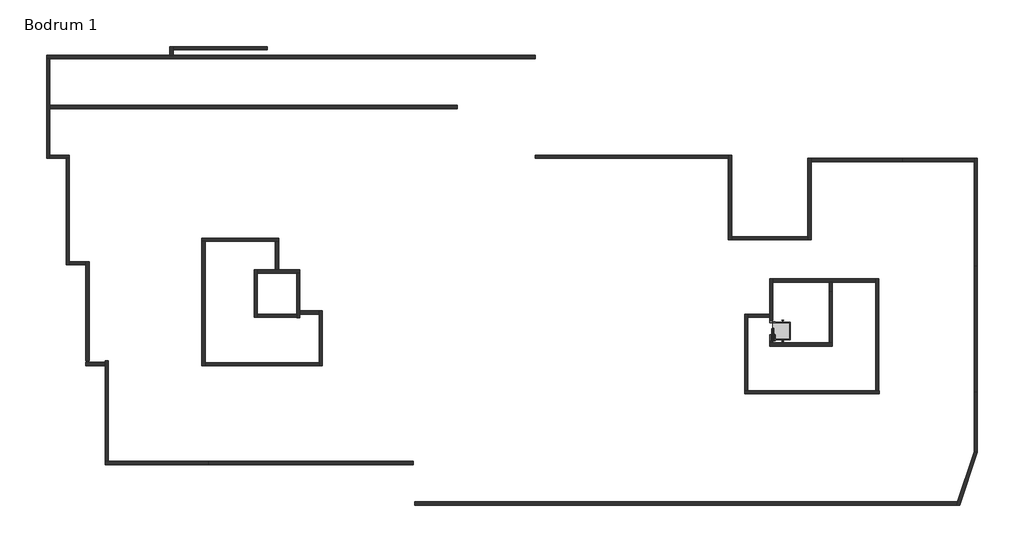
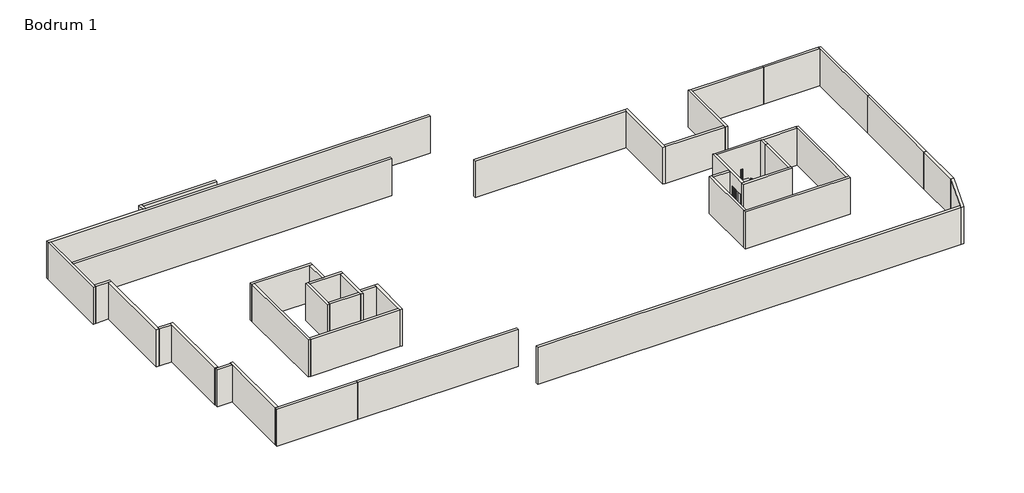
# One storey: 43 walls, 1 proxy.
"""IFC4 building model written with IfcOpenShell, lengths in millimetres."""

import ifcopenshell
import ifcopenshell.guid

model = None  # the IFC model being written
_history = None  # IfcOwnerHistory: only IFC2X3 demands one
_inside = {}  # id of a spatial element -> (the spatial element, [elements in it])
_under = {}  # id of a project, library or spatial element -> (it, [spatial elements below it])
_declared = {}  # id of a project -> (the project, [libraries it declares])
_typed = {}  # id of a type object -> (the type object, [elements of that type])
_made_of = {}  # id of a material, layer set ... -> (it, [elements and type objects made of it])


def new_model(schema):
    """Start an empty IFC model of exactly this schema.

    Asked for "IFC4X3", IfcOpenShell would pick the latest addendum, in which some entities
    have other attributes; the version numbers below select the first issue.
    IFC2X3 requires an IfcOwnerHistory on every rooted entity: one is made here for all.
    """
    global model, _history
    if schema == "IFC4X3":
        model = ifcopenshell.file(schema_version=(4, 3, 0, 0))
    else:
        model = ifcopenshell.file(schema=schema)
    _inside.clear()
    _under.clear()
    _declared.clear()
    _typed.clear()
    _made_of.clear()
    _history = None
    if model.schema == "IFC2X3":
        org = make("IfcOrganization", Name="unknown")
        user = make(
            "IfcPersonAndOrganization",
            ThePerson=make("IfcPerson", FamilyName="unknown"),
            TheOrganization=org,
        )
        app = make(
            "IfcApplication",
            ApplicationDeveloper=org,
            Version="unknown",
            ApplicationFullName="unknown",
            ApplicationIdentifier="unknown",
        )
        _history = make(
            "IfcOwnerHistory",
            OwningUser=user,
            OwningApplication=app,
            ChangeAction="ADDED",
            CreationDate=0,
        )
    return model


def make(cls, **values):
    """One entity of the class cls with the attributes given. An attribute that is None is left unset."""
    return model.create_entity(
        cls, **{name: value for name, value in values.items() if value is not None}
    )


def rooted(cls, **values):
    """An entity with a GlobalId (a new one), such as an element, a storey or a relation."""
    return make(cls, GlobalId=ifcopenshell.guid.new(), OwnerHistory=_history, **values)


def si_unit(unit_type, name, prefix=None):
    """IfcSIUnit, for example si_unit("LENGTHUNIT", "METRE", prefix="MILLI")."""
    return make("IfcSIUnit", UnitType=unit_type, Prefix=prefix, Name=name)


def assignment(units):
    """IfcUnitAssignment: the units of a project."""
    return None if units is None else make("IfcUnitAssignment", Units=units)


def point(xyz):
    """IfcCartesianPoint."""
    return None if xyz is None else make("IfcCartesianPoint", Coordinates=xyz)


def direction(xyz):
    """IfcDirection."""
    return None if xyz is None else make("IfcDirection", DirectionRatios=xyz)


def frame(location, z_axis=None, x_axis=None):
    """IfcAxis2Placement3D, a coordinate frame: its origin and axes. An axis left out is left unset."""
    return make(
        "IfcAxis2Placement3D",
        Location=point(location),
        Axis=direction(z_axis),
        RefDirection=direction(x_axis),
    )


def origin():
    """The frame at (0, 0, 0) with its axes left unset."""
    return frame((0.0, 0.0, 0.0))


def origin_with_axes():
    """The frame at (0, 0, 0) with the z axis (0, 0, 1) and the x axis (1, 0, 0) written out."""
    return frame((0.0, 0.0, 0.0), z_axis=(0.0, 0.0, 1.0), x_axis=(1.0, 0.0, 0.0))


def place(relative_to, where):
    """IfcLocalPlacement: puts the frame where relative to a parent placement (None: the world)."""
    return make(
        "IfcLocalPlacement", PlacementRelTo=relative_to, RelativePlacement=where
    )


def context(
    kind, dimensions, precision=None, world=None, true_north=None, identifier=None
):
    """IfcGeometricRepresentationContext, for example the 3D "Model" context."""
    return make(
        "IfcGeometricRepresentationContext",
        ContextIdentifier=identifier,
        ContextType=kind,
        CoordinateSpaceDimension=dimensions,
        Precision=precision,
        WorldCoordinateSystem=world,
        TrueNorth=true_north,
    )


def project(units=None, contexts=None):
    """IfcProject with its units and contexts."""
    return rooted(
        "IfcProject",
        Name="project",
        RepresentationContexts=contexts,
        UnitsInContext=assignment(units),
    )


def spatial(cls, under=None, at=None, **own):
    """A site, building, storey or space (cls), placed at a placement, below another one or the project."""
    s = rooted(cls, ObjectPlacement=at, **own)
    if under is not None:
        _under.setdefault(under.id(), (under, []))[1].append(s)
    return s


def polyline(points):
    """IfcPolyline through the points."""
    return make("IfcPolyline", Points=[point(p) for p in points])


def outline(outer, holes=None, kind="AREA"):
    """IfcArbitraryClosedProfileDef: a profile drawn as a closed curve; with holes, ...WithVoids."""
    if holes is None:
        return make("IfcArbitraryClosedProfileDef", ProfileType=kind, OuterCurve=outer)
    return make(
        "IfcArbitraryProfileDefWithVoids",
        ProfileType=kind,
        OuterCurve=outer,
        InnerCurves=holes,
    )


def extrude(swept, where, along, depth):
    """IfcExtrudedAreaSolid: the profile swept, set in the frame where, extruded along a direction by depth."""
    return make(
        "IfcExtrudedAreaSolid",
        SweptArea=swept,
        Position=where,
        ExtrudedDirection=direction(along),
        Depth=depth,
    )


def faces_of(points, faces, orient=None, outer=None):
    """IfcFace entities. A face is a list of loops; a loop is a list of indices into points, from 0.

    orient and outer hold one flag for each loop. By default every Orientation is true, the
    first loop of a face is its IfcFaceOuterBound and the others are IfcFaceBound.
    """
    made = []
    for i, loops in enumerate(faces):
        bounds = []
        for j, loop in enumerate(loops):
            is_outer = j == 0 if outer is None else outer[i][j]
            bounds.append(
                make(
                    "IfcFaceOuterBound" if is_outer else "IfcFaceBound",
                    Bound=make("IfcPolyLoop", Polygon=[points[k] for k in loop]),
                    Orientation=True if orient is None else orient[i][j],
                )
            )
        made.append(make("IfcFace", Bounds=bounds))
    return made


def faceted_brep(points, faces, orient=None, outer=None, voids=None):
    """IfcFacetedBrep: a solid bounded by flat faces; with voids (closed shells), ...WithVoids."""
    shared = [point(p) for p in points]
    hull = make("IfcClosedShell", CfsFaces=faces_of(shared, faces, orient, outer))
    if voids is None:
        return make("IfcFacetedBrep", Outer=hull)
    return make(
        "IfcFacetedBrepWithVoids",
        Outer=hull,
        Voids=[
            make(cls, CfsFaces=faces_of(shared, fs, o, b)) for cls, fs, o, b in voids
        ],
    )


def shape(context_of_items, identifier, shape_type, items):
    """IfcShapeRepresentation: the items that make up one representation, for example the "Body"."""
    return make(
        "IfcShapeRepresentation",
        ContextOfItems=context_of_items,
        RepresentationIdentifier=identifier,
        RepresentationType=shape_type,
        Items=items,
    )


def source(mapping_origin, context_of_items, identifier, shape_type, items):
    """IfcRepresentationMap: a shape defined once, which mapped items show again and again."""
    return make(
        "IfcRepresentationMap",
        MappingOrigin=mapping_origin,
        MappedRepresentation=shape(context_of_items, identifier, shape_type, items),
    )


def transform(
    local_origin,
    x_axis=None,
    y_axis=None,
    z_axis=None,
    scale=None,
    scale2=None,
    scale3=None,
    uniform=True,
):
    """IfcCartesianTransformationOperator3D, or its non-uniform kind. x_axis, y_axis, z_axis: its Axis1, 2, 3."""
    if uniform:
        return make(
            "IfcCartesianTransformationOperator3D",
            Axis1=direction(x_axis),
            Axis2=direction(y_axis),
            LocalOrigin=point(local_origin),
            Scale=scale,
            Axis3=direction(z_axis),
        )
    return make(
        "IfcCartesianTransformationOperator3DnonUniform",
        Axis1=direction(x_axis),
        Axis2=direction(y_axis),
        LocalOrigin=point(local_origin),
        Scale=scale,
        Axis3=direction(z_axis),
        Scale2=scale2,
        Scale3=scale3,
    )


def mapped(mapping_source, mapping_target):
    """IfcMappedItem: shows the shape of a source again, moved by a transform."""
    return make(
        "IfcMappedItem", MappingSource=mapping_source, MappingTarget=mapping_target
    )


def made_of(thing, what):
    """Note that an element or type object is made of a material, layer set ...; save() writes the relation."""
    if what is not None:
        _made_of.setdefault(what.id(), (what, []))[1].append(thing)
    return thing


def element(
    cls,
    number,
    at=None,
    inside=None,
    cuts=None,
    type_object=None,
    material=None,
    context=None,
    identifier="Body",
    shape_type=None,
    held_by="IfcProductDefinitionShape",
    body=None,
    shapes=None,
    **own,
):
    """One element of the class cls, such as IfcWall. Its Tag is "e" and its number.

    at: its placement. inside: the storey or other place that contains it. cuts: it is an
    opening in that element (IfcRelVoidsElement). A single representation is given by context,
    identifier, shape_type and body (its items); several are given by shapes. held_by: the class
    of the entity that holds the representations. save() writes the other relations.
    """
    e = rooted(cls, Tag="e%d" % number, ObjectPlacement=at, **own)
    if body is not None:
        shapes = [shape(context, identifier, shape_type, body)]
    if shapes is not None:
        e.Representation = make(held_by, Representations=shapes)
    if inside is not None:
        _inside.setdefault(inside.id(), (inside, []))[1].append(e)
    if cuts is not None:
        rooted(
            "IfcRelVoidsElement", RelatingBuildingElement=cuts, RelatedOpeningElement=e
        )
    if type_object is not None:
        _typed.setdefault(type_object.id(), (type_object, []))[1].append(e)
    return made_of(e, material)


def aggregate(whole, parts):
    """IfcRelAggregates: a whole, such as a stair, and the parts it consists of."""
    return rooted("IfcRelAggregates", RelatingObject=whole, RelatedObjects=parts)


def save(model, path):
    """Write the relations noted so far, then the file.

    IfcRelAggregates (storeys below a building ...), IfcRelContainedInSpatialStructure (elements
    in a storey), IfcRelDefinesByType, IfcRelAssociatesMaterial and IfcRelDeclares: one each for
    every whole, place, type object, material and project.
    """
    for whole, parts in _under.values():
        aggregate(whole, parts)
    for where, things in _inside.values():
        rooted(
            "IfcRelContainedInSpatialStructure",
            RelatedElements=things,
            RelatingStructure=where,
        )
    for kind, things in _typed.values():
        rooted("IfcRelDefinesByType", RelatedObjects=things, RelatingType=kind)
    for what, things in _made_of.values():
        rooted("IfcRelAssociatesMaterial", RelatedObjects=things, RelatingMaterial=what)
    for by, libraries in _declared.values():
        rooted("IfcRelDeclares", RelatingContext=by, RelatedDefinitions=libraries)
    model.write(path)


def m_electric_lift_4_person_wall_based_type_1_25105fba(model_context):
    return source(origin(), model_context, "Body", "SolidModel", [
        extrude(outline(polyline([(-400.0, -1140.0000001), (-400.0, -235.0), (-486.5, -235.0), (-486.5, -105.0), (681.0, -105.0), (681.0, -235.0), (650.0, -235.0), (650.0, -1140.0000001), (-400.0, -1140.0000001)])), frame((0.0, 0.0, 2200.0), z_axis=(0.0, 0.0, 1.0), x_axis=(1.0, 0.0, 0.0)), (0.0, 0.0, 1.0), 22.0),
        extrude(outline(polyline([(-448.6220553, -190.9893804), (-448.6220553, -149.3893804), (-62.6220553, -149.3893804), (-62.6220553, -190.9893804), (-448.6220553, -190.9893804)])), origin_with_axes(), (0.0, 0.0, 1.0), 2000.0),
        extrude(outline(polyline([(-114.8301, -144.0), (-114.8301, -108.9587126), (271.1699, -108.9587126), (271.1699, -144.0), (-114.8301, -144.0)])), origin_with_axes(), (0.0, 0.0, 1.0), 2000.0),
        extrude(outline(polyline([(-488.6220553, 8.3893803), (-102.6220553, 8.3893803), (-102.6220553, -30.6106197), (-488.6220553, -30.6106197), (-488.6220553, 8.3893803)])), origin_with_axes(), (0.0, 0.0, 1.0), 2000.0),
        extrude(outline(polyline([(-124.8301, -75.0), (-124.8301, -36.0), (261.1699, -36.0), (261.1699, -75.0), (-124.8301, -75.0)])), origin_with_axes(), (0.0, 0.0, 1.0), 2000.0),
        extrude(outline(polyline([(-400.0, -1140.0000001), (-400.0, -235.0), (-486.5, -235.0), (-486.5, -105.0), (681.0, -105.0), (681.0, -235.0), (650.0, -235.0), (650.0, -1140.0000001), (-400.0, -1140.0000001)])), frame((0.0, 0.0, -90.0), z_axis=(0.0, 0.0, 1.0), x_axis=(1.0, 0.0, 0.0)), (0.0, 0.0, 1.0), 90.0),
        faceted_brep([(-400.0, -1140.0000001, 2200.0), (650.0, -1140.0000001, 2200.0), (650.0, -235.0, 2200.0), (681.0, -235.0, 2200.0), (681.0, -105.0, 2200.0), (-486.5, -105.0, 2200.0), (-486.5, -235.0, 2200.0), (-400.0, -235.0, 2200.0), (-375.0, -1115.0000001, 2200.0), (-375.0, -235.0, 2200.0), (-110.3, -235.0, 2200.0), (-110.3, -197.0, 2200.0), (-458.1228936, -197.0, 2200.0), (-458.1228936, -108.9587126, 2200.0), (621.1699, -108.9587126, 2200.0), (621.1699, -192.6835257, 2200.0), (600.0, -192.6835257, 2200.0), (600.0, -235.0, 2200.0), (625.0, -235.0, 2200.0), (625.0, -572.5016433, 2200.0), (610.2454439, -572.5016433, 2200.0), (610.2454439, -802.5016433, 2200.0), (625.0, -802.5016433, 2200.0), (625.0, -1115.0000001, 2200.0), (-400.0, -1140.0000001, 0.0), (-400.0, -235.0, 0.0), (-486.5, -235.0, 0.0), (-486.5, -105.0, 0.0), (-173.4437103, -105.0, 0.0), (-173.4437103, -108.9587126, 0.0), (-458.1228936, -108.9587126, 0.0), (-458.1228936, -197.0, 0.0), (-110.3, -197.0, 0.0), (-110.3, -235.0, 0.0), (-375.0, -235.0, 0.0), (-375.0, -1115.0000001, 0.0), (625.0, -1115.0000001, 0.0), (625.0, -802.5016433, 0.0), (610.2454439, -802.5016433, 0.0), (610.2454439, -572.5016433, 0.0), (625.0, -572.5016433, 0.0), (625.0, -235.0, 0.0), (600.0, -235.0, 0.0), (600.0, -192.6835257, 0.0), (621.1699, -192.6835257, 0.0), (621.1699, -105.0, 0.0), (681.0, -105.0, 0.0), (681.0, -235.0, 0.0), (650.0, -235.0, 0.0), (650.0, -1140.0000001, 0.0), (621.1699, -105.0, 2000.0), (-173.4437103, -105.0, 2000.0), (-173.4437103, -108.9587126, 2000.0), (621.1699, -108.9587126, 2000.0), (600.0, -192.6835257, 2000.0)], [[[0, 1, 2, 3, 4, 5, 6, 7], [8, 9, 10, 11, 12, 13, 14, 15, 16, 17, 18, 19, 20, 21, 22, 23]], [[24, 25, 26, 27, 28, 29, 30, 31, 32, 33, 34, 35, 36, 37, 38, 39, 40, 41, 42, 43, 44, 45, 46, 47, 48, 49]], [[1, 0, 24, 49]], [[2, 1, 49, 48]], [[3, 2, 48, 47]], [[4, 3, 47, 46]], [[5, 4, 46, 45, 50, 51, 28, 27]], [[6, 5, 27, 26]], [[7, 6, 26, 25]], [[0, 7, 25, 24]], [[9, 8, 35, 34]], [[10, 9, 34, 33]], [[11, 10, 33, 32]], [[12, 11, 32, 31]], [[13, 12, 31, 30]], [[14, 13, 30, 29, 52, 53]], [[15, 14, 53, 50, 45, 44]], [[16, 15, 44, 43, 54]], [[17, 16, 54, 43, 42]], [[18, 17, 42, 41]], [[19, 18, 41, 40]], [[20, 19, 40, 39]], [[21, 20, 39, 38]], [[22, 21, 38, 37]], [[23, 22, 37, 36]], [[8, 23, 36, 35]], [[50, 53, 52, 51]], [[51, 52, 29, 28]]]),
        extrude(outline(polyline([(750.026988, -751.0012199), (747.026988, -693.80122), (682.0269884, -693.80122), (682.0269884, -681.3056039), (747.1132057, -681.3056039), (750.026988, -624.0012199), (763.026988, -624.0012199), (763.026988, -751.0012199), (750.026988, -751.0012199)])), origin_with_axes(), (0.0, 0.0, 1.0), 3000.0),
        extrude(outline(polyline([(-497.026988, -693.80122), (-500.026988, -751.0012199), (-513.026988, -751.0012199), (-513.026988, -624.0012199), (-500.026988, -624.0012199), (-497.1132057, -681.3056039), (-432.0269884, -681.3056039), (-432.0269884, -693.80122), (-497.026988, -693.80122)])), origin_with_axes(), (0.0, 0.0, 1.0), 3000.0),
        extrude(outline(polyline([(-114.9791786, 100.0), (-114.9791786, 14.4785696), (-505.0067971, 14.4785696), (-505.0067971, 100.0), (-114.9791786, 100.0)])), origin_with_axes(), (0.0, 0.0, 1.0), 2000.0),
        extrude(outline(polyline([(600.0, 5.0), (600.0, 100.0), (750.0, 100.0), (750.0, -75.0), (621.1699, -75.0), (621.1699, 5.0), (600.0, 5.0)])), origin_with_axes(), (0.0, 0.0, 1.0), 2000.0),
    ])


model = new_model("IFC4")

# Units and contexts
model_context = context("Model", 3, world=origin())
ifc_project = project(units=[si_unit("LENGTHUNIT", "METRE", prefix="MILLI")], contexts=[model_context])

# Site, building, storey
site = spatial("IfcSite", under=ifc_project)
building = spatial("IfcBuilding", under=site)
storey = spatial("IfcBuildingStorey", under=building, Name="Bodrum 1", Elevation=-3000.0)

# Proxy
placement = place(None, origin())
m_electric_lift_4_person_wall_based_type_1_shape = m_electric_lift_4_person_wall_based_type_1_25105fba(model_context)
element("IfcBuildingElementProxy", 1, Name="M_Electric Lift-4 person wall based : Type 1", ObjectType="M_Electric Lift-4 person wall based : Type 1", at=placement, inside=storey, context=model_context, shape_type="MappedRepresentation", body=[
    mapped(m_electric_lift_4_person_wall_based_type_1_shape, transform((17860.0831827, -2691.3136213, -3000.0), x_axis=(0.0, 1.0, 0.0), y_axis=(-1.0, 0.0, 0.0), z_axis=(0.0, 0.0, 1.0))),
])

# Walls
element("IfcWall", 2, ObjectType="Generic - 200mm", at=placement, inside=storey, context=model_context, shape_type="SweptSolid", body=[
    extrude(outline(polyline([(30057.8216012, 7604.4428324), (25739.3154183, 7604.4428324), (25739.3154183, 7804.4428324), (30057.8216012, 7804.4428324), (30057.8216012, 7604.4428324)])), frame((0.0, 0.0, -3000.0), z_axis=(0.0, 0.0, 1.0), x_axis=(1.0, 0.0, 0.0)), (0.0, 0.0, 1.0), 3000.0),
])
element("IfcWall", 3, ObjectType="Generic - 200mm", at=placement, inside=storey, context=model_context, shape_type="Brep", body=[
    faceted_brep([(30057.8216012, 7804.4428324, -3000.0), (30057.8216012, 7604.4428324, -3000.0), (30057.8216012, 1304.4428324, -3000.0), (30057.8216012, 1304.4428324, 0.0), (30057.8216012, 7604.4428324, 0.0), (30057.8216012, 7804.4428324, 0.0), (30257.8216012, 7804.4428324, -3000.0), (30257.8216012, 7804.4428324, 0.0), (30257.8216012, 1304.4428324, 0.0), (30257.8216012, 1304.4428324, -3000.0), (30058.3403162, 1304.4428324, -3000.0), (30058.3403162, 1304.4428324, 0.0)], [[[0, 1, 2, 3, 4, 5]], [[6, 7, 8, 9]], [[2, 1, 0, 6, 9, 10]], [[3, 2, 10, 9, 8, 11]], [[5, 4, 3, 11, 8, 7]], [[0, 5, 7, 6]]]),
])
element("IfcWall", 4, ObjectType="Generic - 200mm", at=placement, inside=storey, context=model_context, shape_type="Brep", body=[
    faceted_brep([(30058.3403162, 1304.4428324, -3000.0), (30058.3403162, -6255.0426075, -3000.0), (30058.3403162, -6255.0426075, 0.0), (30058.3403162, 1304.4428324, 0.0), (30258.3403162, 1304.4428324, -3000.0), (30258.3403162, 1304.4428324, 0.0), (30258.3403162, -6255.0426075, 0.0), (30258.3403162, -6255.0426075, -3000.0), (30257.8216012, 1304.4428324, -3000.0), (30058.8590312, -6255.0426075, -3000.0), (30058.8590312, -6255.0426075, 0.0), (30257.8216012, 1304.4428324, 0.0)], [[[0, 1, 2, 3]], [[4, 5, 6, 7]], [[1, 0, 8, 4, 7, 9]], [[2, 1, 9, 7, 6, 10]], [[3, 2, 10, 6, 5, 11]], [[0, 3, 11, 5, 4, 8]]]),
])
element("IfcWall", 5, ObjectType="Generic - 200mm", at=placement, inside=storey, context=model_context, shape_type="Brep", body=[
    faceted_brep([(30058.8590312, -6255.0426075, -3000.0), (30058.8590312, -9846.9059148, -3000.0), (30058.8590312, -9846.9059148, 0.0), (30058.8590312, -6255.0426075, 0.0), (30258.8590312, -6255.0426075, -3000.0), (30258.8590312, -6255.0426075, 0.0), (30258.8590312, -9879.7441648, 0.0), (30258.8590312, -9879.7441648, -3000.0), (30258.3403162, -6255.0426075, -3000.0), (30258.3403162, -6255.0426075, 0.0)], [[[0, 1, 2, 3]], [[4, 5, 6, 7]], [[1, 0, 8, 4, 7]], [[3, 2, 6, 5, 9]], [[0, 3, 9, 5, 4, 8]], [[2, 1, 7, 6]]]),
])
element("IfcWall", 6, ObjectType="Generic - 200mm", at=placement, inside=storey, context=model_context, shape_type="Brep", body=[
    faceted_brep([(21539.3154183, -3291.3136212, -3000.0), (21339.3154183, -3291.3136212, -3000.0), (17960.0831827, -3291.3136212, -3000.0), (17760.0831827, -3291.3136212, -3000.0), (17760.0831827, -3291.3136212, 0.0), (17960.0831827, -3291.3136212, 0.0), (21339.3154183, -3291.3136212, 0.0), (21539.3154183, -3291.3136212, 0.0), (21539.3154183, -3491.3136212, -3000.0), (21539.3154183, -3491.3136212, 0.0), (17760.0831827, -3491.3136212, 0.0), (17760.0831827, -3491.3136212, -3000.0)], [[[0, 1, 2, 3, 4, 5, 6, 7]], [[8, 9, 10, 11]], [[3, 2, 1, 0, 8, 11]], [[7, 6, 5, 4, 10, 9]], [[0, 7, 9, 8]], [[4, 3, 11, 10]]]),
])
element("IfcWall", 7, ObjectType="Generic - 200mm", at=placement, inside=storey, context=model_context, shape_type="SweptSolid", body=[
    extrude(outline(polyline([(-3560.351342, -12851.723579), (29044.7914835, -12851.723579), (28977.2953715, -13051.723579), (-3560.351342, -13051.723579), (-3560.351342, -12851.723579)])), frame((0.0, 0.0, -3000.0), z_axis=(0.0, 0.0, 1.0), x_axis=(1.0, 0.0, 0.0)), (0.0, 0.0, 1.0), 3000.0),
])
element("IfcWall", 8, ObjectType="Generic - 200mm", at=placement, inside=storey, context=model_context, shape_type="Brep", body=[
    faceted_brep([(30058.8590312, -9846.9059148, -3000.0), (29044.7914835, -12851.723579, -3000.0), (28977.2953715, -13051.723579, -3000.0), (28977.2953715, -13051.723579, 0.0), (29044.7914835, -12851.723579, 0.0), (30058.8590312, -9846.9059148, 0.0), (30258.8590312, -9879.7441648, -3000.0), (30258.8590312, -9879.7441648, 0.0), (29188.3776425, -13051.723579, 0.0), (29188.3776425, -13051.723579, -3000.0)], [[[0, 1, 2, 3, 4, 5]], [[6, 7, 8, 9]], [[2, 1, 0, 6, 9]], [[5, 4, 3, 8, 7]], [[0, 5, 7, 6]], [[3, 2, 9, 8]]]),
])
element("IfcWall", 9, ObjectType="Generic - 200mm", at=placement, inside=storey, context=model_context, shape_type="Brep", body=[
    faceted_brep([(24352.8789167, -6155.0426075, -3000.0), (24338.3403162, -6155.0426075, -3000.0), (24138.3403162, -6155.0426075, -3000.0), (16460.0831827, -6155.0426075, -3000.0), (16260.0831827, -6155.0426075, -3000.0), (16260.0831827, -6155.0426075, 0.0), (16460.0831827, -6155.0426075, 0.0), (24138.3403162, -6155.0426075, 0.0), (24338.3403162, -6155.0426075, 0.0), (24352.8789167, -6155.0426075, 0.0), (24352.8789167, -6355.0426075, -3000.0), (24352.8789167, -6355.0426075, 0.0), (16260.0831827, -6355.0426075, 0.0), (16260.0831827, -6355.0426075, -3000.0)], [[[0, 1, 2, 3, 4, 5, 6, 7, 8, 9]], [[10, 11, 12, 13]], [[4, 3, 2, 1, 0, 10, 13]], [[9, 8, 7, 6, 5, 12, 11]], [[0, 9, 11, 10]], [[5, 4, 13, 12]]]),
])
element("IfcWall", 10, ObjectType="Generic - 200mm", at=placement, inside=storey, context=model_context, shape_type="Brep", body=[
    faceted_brep([(24338.3403162, -6155.0426075, -3000.0), (24338.3403162, 564.4428324, -3000.0), (24338.3403162, 564.4428324, 0.0), (24338.3403162, -6155.0426075, 0.0), (24138.3403162, -6155.0426075, -3000.0), (24138.3403162, -6155.0426075, 0.0), (24138.3403162, 364.4428324, 0.0), (24138.3403162, 564.4428324, 0.0), (24138.3403162, 564.4428324, -3000.0), (24138.3403162, 364.4428324, -3000.0)], [[[0, 1, 2, 3]], [[4, 5, 6, 7, 8, 9]], [[1, 0, 4, 9, 8]], [[3, 2, 7, 6, 5]], [[0, 3, 5, 4]], [[2, 1, 8, 7]]]),
])
element("IfcWall", 11, ObjectType="Generic - 200mm", at=placement, inside=storey, context=model_context, shape_type="SweptSolid", body=[
    extrude(outline(polyline([(21339.3154183, -3291.3136212), (21339.3154183, -215.5571676), (21539.3154183, -215.5571676), (21539.3154183, -3291.3136212), (21339.3154183, -3291.3136212)])), frame((0.0, 0.0, -3000.0), z_axis=(0.0, 0.0, 1.0), x_axis=(1.0, 0.0, 0.0)), (0.0, 0.0, 1.0), 3000.0),
])
element("IfcWall", 12, ObjectType="Generic - 200mm", at=placement, inside=storey, context=model_context, shape_type="Brep", body=[
    faceted_brep([(17760.0831827, -3291.3136212, 0.0), (17760.0831827, -1755.0426075, 0.0), (17760.0831827, -1555.0426075, 0.0), (17760.0831827, 564.4428324, 0.0), (17760.0831827, 564.4428324, -3000.0), (17760.0831827, -1555.0426075, -3000.0), (17760.0831827, -1755.0426075, -3000.0), (17760.0831827, -1941.3136213, -3000.0), (17760.0831827, -1941.3136213, -1000.0), (17760.0831827, -3196.3204184, -1000.0), (17760.0831827, -3196.3204184, -3000.0), (17760.0831827, -3291.3136212, -3000.0), (17960.0831827, 564.4428324, 0.0), (17960.0831827, 364.4428324, 0.0), (17960.0831827, -3291.3136212, 0.0), (17960.0831827, -3291.3136212, -3000.0), (17960.0831827, -3196.3204184, -3000.0), (17960.0831827, -3196.3204184, -1000.0), (17960.0831827, -1941.3136213, -1000.0), (17960.0831827, -1941.3136213, -3000.0), (17960.0831827, 364.4428324, -3000.0), (17960.0831827, 564.4428324, -3000.0)], [[[0, 1, 2, 3, 4, 5, 6, 7, 8, 9, 10, 11]], [[12, 13, 14, 15, 16, 17, 18, 19, 20, 21]], [[15, 11, 10, 16]], [[4, 21, 20, 19, 7, 6, 5]], [[3, 2, 1, 0, 14, 13, 12]], [[0, 11, 15, 14]], [[9, 17, 16, 10]], [[18, 8, 7, 19]], [[8, 18, 17, 9]], [[21, 4, 3, 12]]]),
])
element("IfcWall", 13, ObjectType="Generic - 200mm", at=placement, inside=storey, context=model_context, shape_type="SweptSolid", body=[
    extrude(outline(polyline([(21539.3154183, 364.4428324), (21539.3154183, -215.5571676), (21339.3154183, -215.5571676), (21339.3154183, 364.4428324), (21539.3154183, 364.4428324)])), frame((0.0, 0.0, -3000.0), z_axis=(0.0, 0.0, 1.0), x_axis=(1.0, 0.0, 0.0)), (0.0, 0.0, 1.0), 3000.0),
])
element("IfcWall", 14, ObjectType="Generic - 200mm", at=placement, inside=storey, context=model_context, shape_type="SweptSolid", body=[
    extrude(outline(polyline([(25739.3154183, 7604.4428324), (20258.3403162, 7604.4428324), (20258.3403162, 7804.4428324), (25739.3154183, 7804.4428324), (25739.3154183, 7604.4428324)])), frame((0.0, 0.0, -3000.0), z_axis=(0.0, 0.0, 1.0), x_axis=(1.0, 0.0, 0.0)), (0.0, 0.0, 1.0), 3000.0),
])
element("IfcWall", 15, ObjectType="Generic - 200mm", at=placement, inside=storey, context=model_context, shape_type="Brep", body=[
    faceted_brep([(16460.0831827, -6155.0426075, -3000.0), (16460.0831827, -1755.0426075, -3000.0), (16460.0831827, -1555.0426075, -3000.0), (16460.0831827, -1555.0426075, 0.0), (16460.0831827, -1755.0426075, 0.0), (16460.0831827, -6155.0426075, 0.0), (16260.0831827, -6155.0426075, -3000.0), (16260.0831827, -6155.0426075, 0.0), (16260.0831827, -1555.0426075, 0.0), (16260.0831827, -1555.0426075, -3000.0)], [[[0, 1, 2, 3, 4, 5]], [[6, 7, 8, 9]], [[2, 1, 0, 6, 9]], [[5, 4, 3, 8, 7]], [[3, 2, 9, 8]], [[0, 5, 7, 6]]]),
])
element("IfcWall", 16, ObjectType="Generic - 200mm", at=placement, inside=storey, context=model_context, shape_type="Brep", body=[
    faceted_brep([(20058.3403162, 7804.4428324, -3000.0), (20058.3403162, 3104.4428324, -3000.0), (20058.3403162, 2904.4428324, -3000.0), (20058.3403162, 2904.4428324, 0.0), (20058.3403162, 3104.4428324, 0.0), (20058.3403162, 7804.4428324, 0.0), (20258.3403162, 7804.4428324, -3000.0), (20258.3403162, 7804.4428324, 0.0), (20258.3403162, 7604.4428324, 0.0), (20258.3403162, 2904.4428324, 0.0), (20258.3403162, 2904.4428324, -3000.0), (20258.3403162, 7604.4428324, -3000.0)], [[[0, 1, 2, 3, 4, 5]], [[6, 7, 8, 9, 10, 11]], [[2, 1, 0, 6, 11, 10]], [[5, 4, 3, 9, 8, 7]], [[0, 5, 7, 6]], [[3, 2, 10, 9]]]),
])
element("IfcWall", 17, ObjectType="Generic - 200mm", at=placement, inside=storey, context=model_context, shape_type="Brep", body=[
    faceted_brep([(24138.3403162, 564.4428324, -3000.0), (17960.0831827, 564.4428324, -3000.0), (17960.0831827, 564.4428324, 0.0), (24138.3403162, 564.4428324, 0.0), (24138.3403162, 364.4428324, -3000.0), (24138.3403162, 364.4428324, 0.0), (21539.3154183, 364.4428324, 0.0), (21339.3154183, 364.4428324, 0.0), (17960.0831827, 364.4428324, 0.0), (17960.0831827, 364.4428324, -3000.0), (21339.3154183, 364.4428324, -3000.0), (21539.3154183, 364.4428324, -3000.0)], [[[0, 1, 2, 3]], [[4, 5, 6, 7, 8, 9, 10, 11]], [[1, 0, 4, 11, 10, 9]], [[3, 2, 8, 7, 6, 5]], [[2, 1, 9, 8]], [[0, 3, 5, 4]]]),
])
element("IfcWall", 18, ObjectType="Generic - 200mm", at=placement, inside=storey, context=model_context, shape_type="Brep", body=[
    faceted_brep([(-3649.8304233, -10404.1955085, -3000.0), (-15985.351342, -10404.1955085, -3000.0), (-15985.351342, -10404.1955085, 0.0), (-3649.8304233, -10404.1955085, 0.0), (-3649.8304233, -10604.1955085, -3000.0), (-3649.8304233, -10604.1955085, 0.0), (-15985.351342, -10604.1955085, 0.0), (-15985.351342, -10604.1955085, -3000.0), (-15985.351342, -10404.7142235, -3000.0), (-15985.351342, -10404.7142235, 0.0)], [[[0, 1, 2, 3]], [[4, 5, 6, 7]], [[1, 0, 4, 7, 8]], [[2, 1, 8, 7, 6, 9]], [[3, 2, 9, 6, 5]], [[0, 3, 5, 4]]]),
])
element("IfcWall", 19, ObjectType="Generic - 200mm", at=placement, inside=storey, context=model_context, shape_type="Brep", body=[
    faceted_brep([(-15985.351342, -10404.7142235, -3000.0), (-21996.1656446, -10404.7142235, -3000.0), (-22196.1656446, -10404.7142235, -3000.0), (-22196.1656446, -10404.7142235, 0.0), (-21996.1656446, -10404.7142235, 0.0), (-15985.351342, -10404.7142235, 0.0), (-15985.351342, -10604.7142235, -3000.0), (-15985.351342, -10604.7142235, 0.0), (-22196.1656446, -10604.7142235, 0.0), (-22196.1656446, -10604.7142235, -3000.0), (-15985.351342, -10604.1955085, -3000.0), (-15985.351342, -10604.1955085, 0.0)], [[[0, 1, 2, 3, 4, 5]], [[6, 7, 8, 9]], [[2, 1, 0, 10, 6, 9]], [[5, 4, 3, 8, 7, 11]], [[0, 5, 11, 7, 6, 10]], [[3, 2, 9, 8]]]),
])
element("IfcWall", 20, ObjectType="Generic - 200mm", at=placement, inside=storey, context=model_context, shape_type="Brep", body=[
    faceted_brep([(-13036.6223557, -1755.1706106, -3000.0), (-13036.6223557, -1555.1706106, -3000.0), (-13036.6223557, 905.8044915, -3000.0), (-13036.6223557, 1105.8044915, -3000.0), (-13036.6223557, 1105.8044915, 0.0), (-13036.6223557, 905.8044915, 0.0), (-13036.6223557, -1555.1706106, 0.0), (-13036.6223557, -1755.1706106, 0.0), (-13236.6223557, -1755.1706106, -3000.0), (-13236.6223557, -1755.1706106, 0.0), (-13236.6223557, 1105.8044915, 0.0), (-13236.6223557, 1105.8044915, -3000.0)], [[[0, 1, 2, 3, 4, 5, 6, 7]], [[8, 9, 10, 11]], [[3, 2, 1, 0, 8, 11]], [[7, 6, 5, 4, 10, 9]], [[0, 7, 9, 8]], [[4, 3, 11, 10]]]),
])
element("IfcWall", 21, ObjectType="Generic - 200mm", at=placement, inside=storey, context=model_context, shape_type="Brep", body=[
    faceted_brep([(-23157.0323135, -4360.3976601, -3000.0), (-23157.0323135, 1599.6023399, -3000.0), (-23157.0323135, 1599.6023399, 0.0), (-23157.0323135, -4360.3976601, 0.0), (-23357.0323135, -4360.3976601, -3000.0), (-23357.0323135, -4360.3976601, 0.0), (-23357.0323135, 1399.6023399, 0.0), (-23357.0323135, 1599.6023399, 0.0), (-23357.0323135, 1599.6023399, -3000.0), (-23357.0323135, 1399.6023399, -3000.0)], [[[0, 1, 2, 3]], [[4, 5, 6, 7, 8, 9]], [[1, 0, 4, 9, 8]], [[3, 2, 7, 6, 5]], [[0, 3, 5, 4]], [[2, 1, 8, 7]]]),
])
element("IfcWall", 22, ObjectType="Generic - 200mm", at=placement, inside=storey, context=model_context, shape_type="Brep", body=[
    faceted_brep([(-16184.4950909, -4674.1955085, -3000.0), (-16184.4950909, -4474.1955085, -3000.0), (-16184.4950909, 2805.8044915, -3000.0), (-16184.4950909, 2805.8044915, 0.0), (-16184.4950909, -4474.1955085, 0.0), (-16184.4950909, -4674.1955085, 0.0), (-16384.4950909, -4674.1955085, -3000.0), (-16384.4950909, -4674.1955085, 0.0), (-16384.4950909, 2805.8044915, 0.0), (-16384.4950909, 2805.8044915, -3000.0)], [[[0, 1, 2, 3, 4, 5]], [[6, 7, 8, 9]], [[2, 1, 0, 6, 9]], [[5, 4, 3, 8, 7]], [[3, 2, 9, 8]], [[0, 5, 7, 6]]]),
])
element("IfcWall", 23, ObjectType="Generic - 200mm", at=placement, inside=storey, context=model_context, shape_type="SweptSolid", body=[
    extrude(outline(polyline([(-9320.909351, -4674.1955085), (-16184.4950909, -4674.1955085), (-16184.4950909, -4474.1955085), (-9320.909351, -4474.1955085), (-9320.909351, -4674.1955085)])), frame((0.0, 0.0, -3000.0), z_axis=(0.0, 0.0, 1.0), x_axis=(1.0, 0.0, 0.0)), (0.0, 0.0, 1.0), 3000.0),
])
element("IfcWall", 24, ObjectType="Generic - 200mm", at=placement, inside=storey, context=model_context, shape_type="SweptSolid", body=[
    extrude(outline(polyline([(-13036.6223557, -1555.1706106), (-10680.351342, -1555.1706106), (-10680.351342, -1755.1706106), (-13036.6223557, -1755.1706106), (-13036.6223557, -1555.1706106)])), frame((0.0, 0.0, -3000.0), z_axis=(0.0, 0.0, 1.0), x_axis=(1.0, 0.0, 0.0)), (0.0, 0.0, 1.0), 3000.0),
])
element("IfcWall", 25, ObjectType="Generic - 200mm", at=placement, inside=storey, context=model_context, shape_type="Brep", body=[
    faceted_brep([(-10480.351342, 1105.8044915, -3000.0), (-11756.6223557, 1105.8044915, -3000.0), (-11956.6223557, 1105.8044915, -3000.0), (-13036.6223557, 1105.8044915, -3000.0), (-13036.6223557, 1105.8044915, 0.0), (-11956.6223557, 1105.8044915, 0.0), (-11756.6223557, 1105.8044915, 0.0), (-10480.351342, 1105.8044915, 0.0), (-10480.351342, 905.8044915, -3000.0), (-10480.351342, 905.8044915, 0.0), (-10680.351342, 905.8044915, 0.0), (-13036.6223557, 905.8044915, 0.0), (-13036.6223557, 905.8044915, -3000.0), (-10680.351342, 905.8044915, -3000.0)], [[[0, 1, 2, 3, 4, 5, 6, 7]], [[8, 9, 10, 11, 12, 13]], [[3, 2, 1, 0, 8, 13, 12]], [[7, 6, 5, 4, 11, 10, 9]], [[0, 7, 9, 8]], [[4, 3, 12, 11]]]),
])
element("IfcWall", 26, ObjectType="Generic - 200mm", at=placement, inside=storey, context=model_context, shape_type="Brep", body=[
    faceted_brep([(-10480.351342, -1794.1955085, -3000.0), (-10480.351342, -1555.1706106, -3000.0), (-10480.351342, -1355.1706106, -3000.0), (-10480.351342, 905.8044915, -3000.0), (-10480.351342, 905.8044915, 0.0), (-10480.351342, -1355.1706106, 0.0), (-10480.351342, -1555.1706106, 0.0), (-10480.351342, -1794.1955085, 0.0), (-10680.351342, -1794.1955085, -3000.0), (-10680.351342, -1794.1955085, 0.0), (-10680.351342, -1755.1706106, 0.0), (-10680.351342, -1555.1706106, 0.0), (-10680.351342, 905.8044915, 0.0), (-10680.351342, 905.8044915, -3000.0), (-10680.351342, -1555.1706106, -3000.0), (-10680.351342, -1755.1706106, -3000.0)], [[[0, 1, 2, 3, 4, 5, 6, 7]], [[8, 9, 10, 11, 12, 13, 14, 15]], [[3, 2, 1, 0, 8, 15, 14, 13]], [[7, 6, 5, 4, 12, 11, 10, 9]], [[0, 7, 9, 8]], [[4, 3, 13, 12]]]),
])
element("IfcWall", 27, ObjectType="Generic - 200mm", at=placement, inside=storey, context=model_context, shape_type="SweptSolid", body=[
    extrude(outline(polyline([(-18100.351342, 14525.8044915), (-12436.6223557, 14525.8044915), (-12436.6223557, 14325.8044915), (-18100.351342, 14325.8044915), (-18100.351342, 14525.8044915)])), frame((0.0, 0.0, -3000.0), z_axis=(0.0, 0.0, 1.0), x_axis=(1.0, 0.0, 0.0)), (0.0, 0.0, 1.0), 3000.0),
])
element("IfcWall", 28, ObjectType="Generic - 200mm", at=placement, inside=storey, context=model_context, shape_type="Brep", body=[
    faceted_brep([(-25711.9578682, 13797.8072329, -3000.0), (-25711.9578682, 7797.8072329, -3000.0), (-25711.9578682, 7797.8072329, 0.0), (-25711.9578682, 13797.8072329, 0.0), (-25511.9578682, 13797.8072329, -3000.0), (-25511.9578682, 13797.8072329, 0.0), (-25511.9578682, 10997.8072329, 0.0), (-25511.9578682, 10797.8072329, 0.0), (-25511.9578682, 7997.8072329, 0.0), (-25511.9578682, 7797.8072329, 0.0), (-25511.9578682, 7797.8072329, -3000.0), (-25511.9578682, 7997.8072329, -3000.0), (-25511.9578682, 10797.8072329, -3000.0), (-25511.9578682, 10997.8072329, -3000.0)], [[[0, 1, 2, 3]], [[4, 5, 6, 7, 8, 9, 10, 11, 12, 13]], [[1, 0, 4, 13, 12, 11, 10]], [[3, 2, 9, 8, 7, 6, 5]], [[2, 1, 10, 9]], [[0, 3, 5, 4]]]),
])
element("IfcWall", 29, ObjectType="Generic - 200mm", at=placement, inside=storey, context=model_context, shape_type="Brep", body=[
    faceted_brep([(-25511.9578682, 7797.8072329, -3000.0), (-24534.4950909, 7797.8072329, -3000.0), (-24334.4950909, 7797.8072329, -3000.0), (-24334.4950909, 7797.8072329, 0.0), (-24534.4950909, 7797.8072329, 0.0), (-25511.9578682, 7797.8072329, 0.0), (-25511.9578682, 7997.8072329, -3000.0), (-25511.9578682, 7997.8072329, 0.0), (-24334.4950909, 7997.8072329, 0.0), (-24334.4950909, 7997.8072329, -3000.0)], [[[0, 1, 2, 3, 4, 5]], [[6, 7, 8, 9]], [[2, 1, 0, 6, 9]], [[5, 4, 3, 8, 7]], [[0, 5, 7, 6]], [[3, 2, 9, 8]]]),
])
element("IfcWall", 30, ObjectType="Generic - 200mm", at=placement, inside=storey, context=model_context, shape_type="Brep", body=[
    faceted_brep([(3678.3403162, 13997.8072329, -3000.0), (-18100.351342, 13997.8072329, -3000.0), (-18300.351342, 13997.8072329, -3000.0), (-25711.9578682, 13997.8072329, -3000.0), (-25711.9578682, 13997.8072329, 0.0), (-18300.351342, 13997.8072329, 0.0), (-18100.351342, 13997.8072329, 0.0), (3678.3403162, 13997.8072329, 0.0), (3678.3403162, 13797.8072329, -3000.0), (3678.3403162, 13797.8072329, 0.0), (-25511.9578682, 13797.8072329, 0.0), (-25711.9578682, 13797.8072329, 0.0), (-25711.9578682, 13797.8072329, -3000.0), (-25511.9578682, 13797.8072329, -3000.0)], [[[0, 1, 2, 3, 4, 5, 6, 7]], [[8, 9, 10, 11, 12, 13]], [[3, 2, 1, 0, 8, 13, 12]], [[7, 6, 5, 4, 11, 10, 9]], [[0, 7, 9, 8]], [[4, 3, 12, 11]]]),
])
element("IfcWall", 31, ObjectType="Generic - 200mm", at=placement, inside=storey, context=model_context, shape_type="Brep", body=[
    faceted_brep([(-24534.4950909, 7797.8072329, -3000.0), (-24534.4950909, 1399.6023399, -3000.0), (-24534.4950909, 1399.6023399, 0.0), (-24534.4950909, 7797.8072329, 0.0), (-24334.4950909, 7797.8072329, -3000.0), (-24334.4950909, 7797.8072329, 0.0), (-24334.4950909, 1599.6023399, 0.0), (-24334.4950909, 1399.6023399, 0.0), (-24334.4950909, 1399.6023399, -3000.0), (-24334.4950909, 1599.6023399, -3000.0)], [[[0, 1, 2, 3]], [[4, 5, 6, 7, 8, 9]], [[1, 0, 4, 9, 8]], [[3, 2, 7, 6, 5]], [[0, 3, 5, 4]], [[2, 1, 8, 7]]]),
])
element("IfcWall", 32, ObjectType="Generic - 200mm", at=placement, inside=storey, context=model_context, shape_type="Brep", body=[
    faceted_brep([(-21996.1656446, -10404.7142235, -3000.0), (-21996.1656446, -4360.3976601, -3000.0), (-21996.1656446, -4360.3976601, 0.0), (-21996.1656446, -10404.7142235, 0.0), (-22196.1656446, -10404.7142235, -3000.0), (-22196.1656446, -10404.7142235, 0.0), (-22196.1656446, -4660.3976601, 0.0), (-22196.1656446, -4460.3976601, 0.0), (-22196.1656446, -4360.3976601, 0.0), (-22196.1656446, -4360.3976601, -3000.0), (-22196.1656446, -4460.3976601, -3000.0), (-22196.1656446, -4660.3976601, -3000.0)], [[[0, 1, 2, 3]], [[4, 5, 6, 7, 8, 9, 10, 11]], [[1, 0, 4, 11, 10, 9]], [[2, 1, 9, 8]], [[3, 2, 8, 7, 6, 5]], [[0, 3, 5, 4]]]),
])
element("IfcWall", 33, ObjectType="Generic - 200mm", at=placement, inside=storey, context=model_context, shape_type="Brep", body=[
    faceted_brep([(-16384.4950909, 2805.8044915, -3000.0), (-16184.4950909, 2805.8044915, -3000.0), (-11956.6223557, 2805.8044915, -3000.0), (-11756.6223557, 2805.8044915, -3000.0), (-11756.6223557, 2805.8044915, 0.0), (-11956.6223557, 2805.8044915, 0.0), (-16184.4950909, 2805.8044915, 0.0), (-16384.4950909, 2805.8044915, 0.0), (-16384.4950909, 3005.8044915, -3000.0), (-16384.4950909, 3005.8044915, 0.0), (-11756.6223557, 3005.8044915, 0.0), (-11756.6223557, 3005.8044915, -3000.0)], [[[0, 1, 2, 3, 4, 5, 6, 7]], [[8, 9, 10, 11]], [[3, 2, 1, 0, 8, 11]], [[7, 6, 5, 4, 10, 9]], [[0, 7, 9, 8]], [[4, 3, 11, 10]]]),
])
element("IfcWall", 34, ObjectType="Generic - 200mm", at=placement, inside=storey, context=model_context, shape_type="Brep", body=[
    faceted_brep([(-9320.909351, -1355.1706106, -3000.0), (-9320.909351, -1555.1706106, -3000.0), (-9320.909351, -4474.1955085, -3000.0), (-9320.909351, -4674.1955085, -3000.0), (-9320.909351, -4674.1955085, 0.0), (-9320.909351, -4474.1955085, 0.0), (-9320.909351, -1555.1706106, 0.0), (-9320.909351, -1355.1706106, 0.0), (-9120.909351, -1355.1706106, -3000.0), (-9120.909351, -1355.1706106, 0.0), (-9120.909351, -4674.1955085, 0.0), (-9120.909351, -4674.1955085, -3000.0)], [[[0, 1, 2, 3, 4, 5, 6, 7]], [[8, 9, 10, 11]], [[3, 2, 1, 0, 8, 11]], [[7, 6, 5, 4, 10, 9]], [[0, 7, 9, 8]], [[4, 3, 11, 10]]]),
])
element("IfcWall", 35, ObjectType="Generic - 200mm", at=placement, inside=storey, context=model_context, shape_type="SweptSolid", body=[
    extrude(outline(polyline([(20058.3403162, 2904.4428324), (15478.3403162, 2904.4428324), (15478.3403162, 3104.4428324), (20058.3403162, 3104.4428324), (20058.3403162, 2904.4428324)])), frame((0.0, 0.0, -3000.0), z_axis=(0.0, 0.0, 1.0), x_axis=(1.0, 0.0, 0.0)), (0.0, 0.0, 1.0), 3000.0),
])
element("IfcWall", 36, ObjectType="Generic - 200mm", at=placement, inside=storey, context=model_context, shape_type="Brep", body=[
    faceted_brep([(15478.3403162, 2904.4428324, -3000.0), (15478.3403162, 3104.4428324, -3000.0), (15478.3403162, 8004.4428324, -3000.0), (15478.3403162, 8004.4428324, 0.0), (15478.3403162, 3104.4428324, 0.0), (15478.3403162, 2904.4428324, 0.0), (15278.3403162, 2904.4428324, -3000.0), (15278.3403162, 2904.4428324, 0.0), (15278.3403162, 7804.4428324, 0.0), (15278.3403162, 8004.4428324, 0.0), (15278.3403162, 8004.4428324, -3000.0), (15278.3403162, 7804.4428324, -3000.0)], [[[0, 1, 2, 3, 4, 5]], [[6, 7, 8, 9, 10, 11]], [[2, 1, 0, 6, 11, 10]], [[5, 4, 3, 9, 8, 7]], [[3, 2, 10, 9]], [[0, 5, 7, 6]]]),
])
element("IfcWall", 37, ObjectType="Generic - 200mm", at=placement, inside=storey, context=model_context, shape_type="SweptSolid", body=[
    extrude(outline(polyline([(3678.3403162, 8004.4428324), (15278.3403162, 8004.4428324), (15278.3403162, 7804.4428324), (3678.3403162, 7804.4428324), (3678.3403162, 8004.4428324)])), frame((0.0, 0.0, -3000.0), z_axis=(0.0, 0.0, 1.0), x_axis=(1.0, 0.0, 0.0)), (0.0, 0.0, 1.0), 3000.0),
])
element("IfcWall", 38, ObjectType="Generic - 200mm", at=placement, inside=storey, context=model_context, shape_type="SweptSolid", body=[
    extrude(outline(polyline([(-10480.351342, -1355.1706106), (-9320.909351, -1355.1706106), (-9320.909351, -1555.1706106), (-10480.351342, -1555.1706106), (-10480.351342, -1355.1706106)])), frame((0.0, 0.0, -3000.0), z_axis=(0.0, 0.0, 1.0), x_axis=(1.0, 0.0, 0.0)), (0.0, 0.0, 1.0), 3000.0),
])
element("IfcWall", 39, ObjectType="Generic - 200mm", at=placement, inside=storey, context=model_context, shape_type="Brep", body=[
    faceted_brep([(-18100.351342, 13997.8072329, -3000.0), (-18100.351342, 14325.8044915, -3000.0), (-18100.351342, 14525.8044915, -3000.0), (-18100.351342, 14525.8044915, 0.0), (-18100.351342, 14325.8044915, 0.0), (-18100.351342, 13997.8072329, 0.0), (-18300.351342, 13997.8072329, -3000.0), (-18300.351342, 13997.8072329, 0.0), (-18300.351342, 14525.8044915, 0.0), (-18300.351342, 14525.8044915, -3000.0)], [[[0, 1, 2, 3, 4, 5]], [[6, 7, 8, 9]], [[2, 1, 0, 6, 9]], [[5, 4, 3, 8, 7]], [[3, 2, 9, 8]], [[0, 5, 7, 6]]]),
])
element("IfcWall", 40, ObjectType="Generic - 200mm", at=placement, inside=storey, context=model_context, shape_type="SweptSolid", body=[
    extrude(outline(polyline([(17760.0831827, -1755.0426075), (16460.0831827, -1755.0426075), (16460.0831827, -1555.0426075), (17760.0831827, -1555.0426075), (17760.0831827, -1755.0426075)])), frame((0.0, 0.0, -3000.0), z_axis=(0.0, 0.0, 1.0), x_axis=(1.0, 0.0, 0.0)), (0.0, 0.0, 1.0), 3000.0),
])
element("IfcWall", 41, ObjectType="Generic - 200mm", at=placement, inside=storey, context=model_context, shape_type="SweptSolid", body=[
    extrude(outline(polyline([(-22196.1656446, -4660.3976601), (-23357.0323135, -4660.3976601), (-23357.0323135, -4460.3976601), (-22196.1656446, -4460.3976601), (-22196.1656446, -4660.3976601)])), frame((0.0, 0.0, -3000.0), z_axis=(0.0, 0.0, 1.0), x_axis=(1.0, 0.0, 0.0)), (0.0, 0.0, 1.0), 3000.0),
])
element("IfcWall", 42, ObjectType="Generic - 200mm", at=placement, inside=storey, context=model_context, shape_type="SweptSolid", body=[
    extrude(outline(polyline([(-24334.4950909, 1599.6023399), (-23357.0323135, 1599.6023399), (-23357.0323135, 1399.6023399), (-24334.4950909, 1399.6023399), (-24334.4950909, 1599.6023399)])), frame((0.0, 0.0, -3000.0), z_axis=(0.0, 0.0, 1.0), x_axis=(1.0, 0.0, 0.0)), (0.0, 0.0, 1.0), 3000.0),
])
element("IfcWall", 43, ObjectType="Generic - 200mm", at=placement, inside=storey, context=model_context, shape_type="SweptSolid", body=[
    extrude(outline(polyline([(-11756.6223557, 2805.8044915), (-11756.6223557, 1105.8044915), (-11956.6223557, 1105.8044915), (-11956.6223557, 2805.8044915), (-11756.6223557, 2805.8044915)])), frame((0.0, 0.0, -3000.0), z_axis=(0.0, 0.0, 1.0), x_axis=(1.0, 0.0, 0.0)), (0.0, 0.0, 1.0), 3000.0),
])
element("IfcWall", 44, ObjectType="Generic - 200mm", at=placement, inside=storey, context=model_context, shape_type="SweptSolid", body=[
    extrude(outline(polyline([(-25511.9578682, 10997.8072329), (-1011.9578682, 10997.8072329), (-1011.9578682, 10797.8072329), (-25511.9578682, 10797.8072329), (-25511.9578682, 10997.8072329)])), frame((0.0, 0.0, -3000.0), z_axis=(0.0, 0.0, 1.0), x_axis=(1.0, 0.0, 0.0)), (0.0, 0.0, 1.0), 3000.0),
])

save(model, "model.ifc")

# Revit data of these elements
# Project information
#   Project Issue Date = "Issue Date"
#   Project Status = "Project Status"
#   Client Name = "Owner"
#   Project Address = "Enter address here"
#   Project Name = "Project Name"
#   Project Number = "0001"
# Type "M_Electric Lift-4 person wall based : Type 1"
#   Door Material = none
#   Manufacturer = ""
#   Default Elevation = 0
#   Assembly Code = ""
# Type "Generic - 200mm"
#   Layers, outside or top first: 20 cm no material (function 1)
# Element 1 (IfcBuildingElementProxy, "M_Electric Lift-4 person wall based : Type 1")
#   Phase Created = New Construction
# Elements 2, 3, 4, 5, 6, 7, 8, 9, 10, 11, 12, 13, 14, 15, 16, 17, 18, 19, 20, 21, 22, 23, 24, 25, 26, 27, 28, 29, 30, 31, 32, 33, 34, 35, 36, 37, 38, 39, 40, 41, 42, 43, 44 (IfcWall, "Generic - 200mm")
#   Top Offset = 0 cm
#   Base Offset = 0 cm
#   wall height = 300 cm
#   Phase Created = New Construction
#   Base Constraint = Bodrum 1
#   Top Constraint = Zemin
#   Materials on its faces: "Default Wall"
# Materials
#   "Default Wall": class "Miscellaneous", colour RGB 128 128 128, transparency 0, Cost = 0
